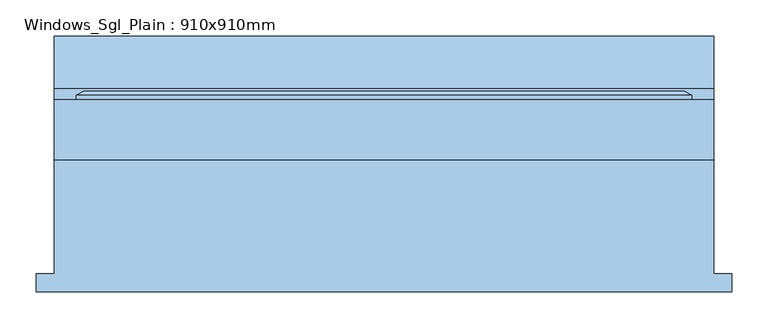
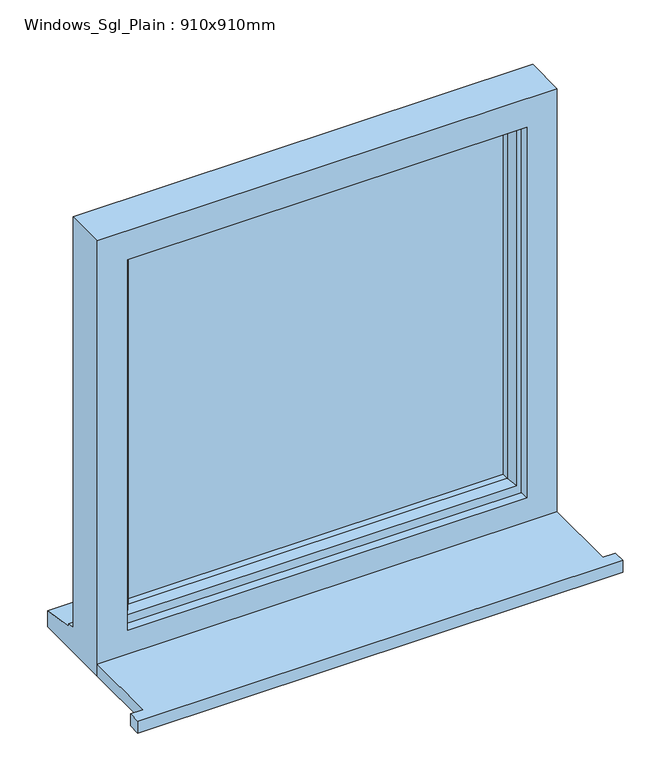
"""IFC4 building model written with IfcOpenShell, lengths in millimetres: window geometry, Windows_Sgl_Plain : 910x910mm."""

from ifc_helpers import new_model, si_unit, frame, origin, place, context, project, spatial, polyline, outline, extrude, faceted_brep, source, transform, mapped, element, save


def windows_sgl_plain_910x910mm_b9caa461(model_context):
    return source(origin(), model_context, "Body", "SolidModel", [
        extrude(outline(polyline([(-480.0, -161.5434322), (-480.0, -136.5434322), (-455.0, -136.5434322), (-455.0, 20.4565678), (455.0, 20.4565678), (455.0, -136.5434322), (480.0, -136.5434322), (480.0, -161.5434322), (-480.0, -161.5434322)])), frame((0.0, 0.0, 1200.0), z_axis=(0.0, 0.0, 1.0), x_axis=(1.0, 0.0, 0.0)), (0.0, 0.0, 1.0), 25.0),
        faceted_brep([(-455.0, 20.4565678, 1200.0), (455.0, 20.4565678, 1200.0), (455.0, 20.4565678, 2110.0), (-455.0, 20.4565678, 2110.0), (-395.0, 20.4565678, 2050.0), (395.0, 20.4565678, 2050.0), (395.0, 20.4565678, 1275.0), (-395.0, 20.4565678, 1275.0), (-455.0, 103.4565678, 2110.0), (-455.0, 103.4565678, 1251.0), (-455.0, 118.4565678, 1249.68767), (-455.0, 118.4565678, 1244.7449676), (-455.0, 190.9565678, 1233.8088847), (-455.0, 190.9565678, 1200.0), (455.0, 103.4565678, 2110.0), (455.0, 103.4565678, 1251.0), (-415.0, 103.4565678, 2070.0), (-415.0, 103.4565678, 1263.0), (415.0, 103.4565678, 1263.0), (415.0, 103.4565678, 2070.0), (-415.0, 38.4565678, 2070.0), (-415.0, 38.4565678, 1263.0), (415.0, 38.4565678, 2070.0), (415.0, 38.4565678, 1263.0), (-395.0, 38.4565678, 2050.0), (-395.0, 38.4565678, 1275.0), (395.0, 38.4565678, 1275.0), (395.0, 38.4565678, 2050.0), (455.0, 190.9565678, 1200.0), (455.0, 190.9565678, 1233.8088847), (455.0, 118.4565678, 1244.7449676), (455.0, 118.4565678, 1249.68767)], [[[0, 1, 2, 3], [4, 5, 6, 7]], [[0, 3, 8, 9, 10, 11, 12, 13]], [[9, 8, 14, 15], [16, 17, 18, 19]], [[17, 16, 20, 21]], [[20, 22, 23, 21], [24, 25, 26, 27]], [[24, 4, 7, 25]], [[3, 2, 14, 8]], [[16, 19, 22, 20]], [[5, 4, 24, 27]], [[15, 14, 2, 1, 28, 29, 30, 31]], [[19, 18, 23, 22]], [[5, 27, 26, 6]], [[28, 1, 0, 13]], [[29, 28, 13, 12]], [[30, 29, 12, 11]], [[31, 30, 11, 10]], [[15, 31, 10, 9]], [[21, 23, 18, 17]], [[7, 6, 26, 25]]]),
        extrude(outline(polyline([(385.0, 67.4565678), (-385.0, 67.4565678), (-385.0, 91.4565678), (385.0, 91.4565678), (385.0, 67.4565678)])), frame((0.0, 0.0, 1293.0), z_axis=(0.0, 0.0, 1.0), x_axis=(1.0, 0.0, 0.0)), (0.0, 0.0, 1.0), 747.0),
        faceted_brep([(-425.0, 103.4565678, 2080.0), (-425.0, 109.2300705, 2080.0), (-425.0, 109.2300705, 1253.0), (-425.0, 103.4565678, 1253.0), (-415.0, 38.4565678, 2070.0), (-415.0, 103.4565678, 2070.0), (-415.0, 103.4565678, 1263.0), (-415.0, 38.4565678, 1263.0), (-375.0, 52.9494677, 2030.0), (-385.1480377, 38.4565678, 2040.1480377), (-385.1480377, 38.4565678, 1292.8519623), (-375.0, 52.9494677, 1303.0), (-375.0, 67.4565678, 2030.0), (-375.0, 67.4565678, 1303.0), (-385.0, 91.4565678, 2040.0), (-385.0, 67.4565678, 2040.0), (-385.0, 67.4565678, 1293.0), (-385.0, 91.4565678, 1293.0), (-375.0, 109.2300705, 2030.0), (-375.0, 91.4565678, 2030.0), (-375.0, 91.4565678, 1303.0), (-375.0, 109.2300705, 1303.0), (-392.4457548, 115.0035732, 2047.4457548), (-392.4457548, 115.0035732, 1285.5542452), (-414.2153903, 115.0035732, 2069.2153903), (-414.2153903, 115.0035732, 1263.7846097), (425.0, 109.2300705, 1253.0), (425.0, 103.4565678, 1253.0), (415.0, 103.4565678, 1263.0), (415.0, 38.4565678, 1263.0), (385.1480377, 38.4565678, 1292.8519623), (375.0, 52.9494677, 1303.0), (375.0, 67.4565678, 1303.0), (385.0, 67.4565678, 1293.0), (385.0, 91.4565678, 1293.0), (375.0, 91.4565678, 1303.0), (375.0, 109.2300705, 1303.0), (392.4457548, 115.0035732, 1285.5542452), (414.2153903, 115.0035732, 1263.7846097), (425.0, 109.2300705, 2080.0), (425.0, 103.4565678, 2080.0), (415.0, 103.4565678, 2070.0), (415.0, 38.4565678, 2070.0), (385.1480377, 38.4565678, 2040.1480377), (375.0, 52.9494677, 2030.0), (375.0, 67.4565678, 2030.0), (385.0, 67.4565678, 2040.0), (385.0, 91.4565678, 2040.0), (375.0, 91.4565678, 2030.0), (375.0, 109.2300705, 2030.0), (392.4457548, 115.0035732, 2047.4457548), (414.2153903, 115.0035732, 2069.2153903)], [[[0, 1, 2, 3]], [[4, 5, 6, 7]], [[8, 9, 10, 11]], [[12, 8, 11, 13]], [[14, 15, 16, 17]], [[18, 19, 20, 21]], [[22, 18, 21, 23]], [[1, 24, 25, 2]], [[3, 2, 26, 27]], [[7, 6, 28, 29]], [[11, 10, 30, 31]], [[13, 11, 31, 32]], [[17, 16, 33, 34]], [[21, 20, 35, 36]], [[23, 21, 36, 37]], [[2, 25, 38, 26]], [[27, 26, 39, 40]], [[29, 28, 41, 42]], [[31, 30, 43, 44]], [[32, 31, 44, 45]], [[34, 33, 46, 47]], [[36, 35, 48, 49]], [[37, 36, 49, 50]], [[26, 38, 51, 39]], [[40, 39, 1, 0]], [[3, 27, 40, 0], [5, 41, 28, 6]], [[42, 41, 5, 4]], [[7, 29, 42, 4], [9, 43, 30, 10]], [[44, 43, 9, 8]], [[45, 44, 8, 12]], [[15, 46, 33, 16], [13, 32, 45, 12]], [[47, 46, 15, 14]], [[17, 34, 47, 14], [19, 48, 35, 20]], [[49, 48, 19, 18]], [[50, 49, 18, 22]], [[24, 51, 38, 25], [23, 37, 50, 22]], [[39, 51, 24, 1]]]),
    ])


if __name__ == "__main__":
    model = new_model("IFC4")
    model_context = context("Model", 3, world=origin())
    ifc_project = project(units=[si_unit("LENGTHUNIT", "METRE", prefix="MILLI")], contexts=[model_context])
    site = spatial("IfcSite", under=ifc_project)
    building = spatial("IfcBuilding", under=site)
    placement = place(None, origin())
    windows_sgl_plain_910x910mm_shape = windows_sgl_plain_910x910mm_b9caa461(model_context)
    element("IfcWindow", 1, ObjectType="Windows_Sgl_Plain : 910x910mm", at=placement, inside=building, context=model_context, shape_type="MappedRepresentation", body=[
        mapped(windows_sgl_plain_910x910mm_shape, transform((0.0, 0.0, 0.0), x_axis=(1.0, 0.0, 0.0), y_axis=(0.0, 1.0, 0.0), z_axis=(0.0, 0.0, 1.0))),
    ])
    save(model, "model.ifc")

# Revit data of these elements
# Type "Windows_Sgl_Plain : 910x910mm"
#   Type Mark = "44"
#   Operation = "SinglePanel"
#   Construction Type Id = "SGL"
#   Manufacturer = "Revit"
#   Keynote = "L10"
#   Analytic Construction = "Large single-glazed windows"
#   Wrap Layers (Ext) from Ext = 102.5 mm
#   Wrap Layers (Int) from Ext = 177.5 mm
#   Window Board Projection = 25 mm
#   Window Board Extension = 25 mm
#   Visual Light Transmittance = 0.9
#   Solar Heat Gain Coefficient = 0.86
#   Rough Width = 910 mm
#   Rough Height = 910 mm
#   Height = 910 mm
#   Width = 910 mm
#   Heat Transfer Coefficient (U) = 5.5617 W/(m²·K)
#   Glazing Thickness = 24 mm
#   FrameOffset - External = 50 mm
#   Frame Depth = 65 mm
#   Default Head Height = 2110 mm
#   Cill Depth = 87.5 mm
#   Cavity Closer Width = 50 mm
#   Cavity Closer Offset from Ext = 102.5 mm
#   Cavity Closer Depth = 85 mm
#   Define Thermal Properties by = 1
#   Vis - Cavity Closers = yes
#   Define Thermal Properties by = 1
#   Material Trim = Window Frame
#   Material Glass = Glass
#   Material Frame = Window Frame
#   Wall Closure = (empty or 0)
# Element 1 (IfcWindow, "Windows_Sgl_Plain : 910x910mm")
#   Materials on its faces: "Window Frame", "Glass"
# Materials
#   "Window Frame": class "Miscellaneous", colour RGB 249 249 249, transparency 0, Keynote = "L10", Cost = 0
#   "Glass": class "Glass", colour RGB 0 128 192, transparency 0.9, Description = "Soda Lime Glass", Cost = 0
